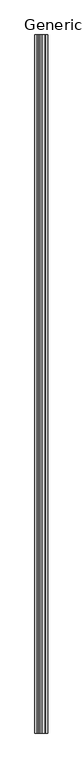
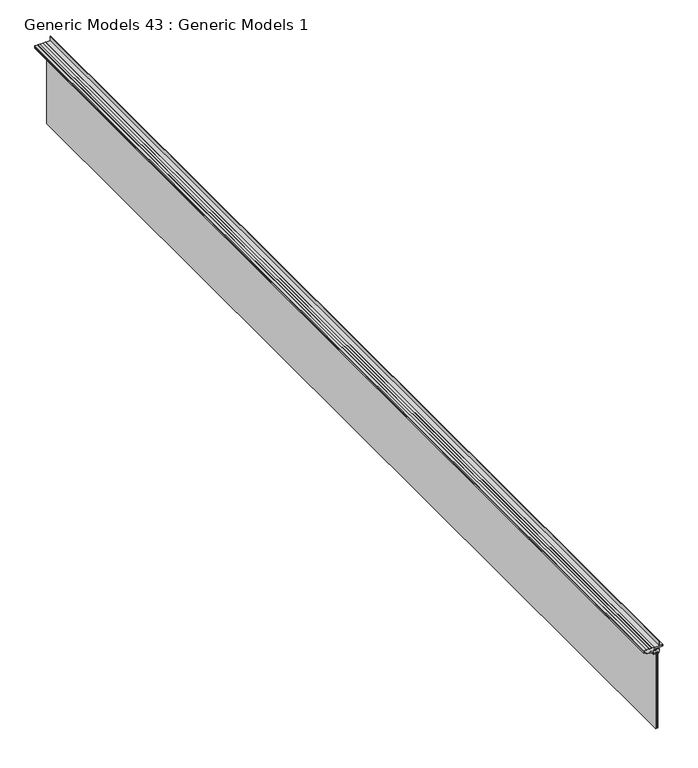
"""IFC4 building model written with IfcOpenShell, lengths in millimetres: proxy geometry, Generic Models 43 : Generic Models 1."""

from ifc_helpers import new_model, si_unit, point, frame, frame_2d, origin, place, context, project, spatial, polyline, circle_curve, trimmed, segment, composite_curve, outline, extrude, source, transform, mapped, element, save


def generic_models_43_generic_models_1_91aa61af(model_context):
    return source(origin(), model_context, "Body", "SweptSolid", [
        extrude(outline(composite_curve([segment(polyline([(126196.7118395, 4830.4400913), (126188.7616223, 4830.4400913), (126188.7616223, 4838.3902843), (126186.7804448, 4838.3902843), (126186.7804448, 4830.4400913), (126176.8490258, 4830.4400913), (126176.8490258, 4840.7524463), (126176.0362363, 4841.5398982), (126176.0362363, 4844.7148982), (126172.0738328, 4844.7148982), (126172.0738328, 4846.3150913), (126168.8988328, 4850.2520602), (126168.8988328, 4851.8522533), (126166.5112363, 4851.8522533), (126166.5112363, 4870.9022533), (126160.1794038, 4870.9022533), (126160.1794038, 4900.3154773), (126163.3544038, 4900.3154773), (126163.3544038, 4897.2675044), (126172.0412038, 4897.2675044), (126172.0412038, 4879.7415044), (126174.3272038, 4879.7415044), (126174.3272038, 4897.2675044), (126175.2670003, 4897.2675044), (126175.2670003, 4905.6748401), (126183.2171933, 4905.6748401), (126183.2171933, 4907.6561145), (126176.7982537, 4907.6561145), (126176.7982537, 4911.6692416), (126181.6750463, 4911.6692416), (126181.6750463, 4946.6196416), (126184.0974162, 4974.4834416), (126193.0288395, 4974.4834416), (126193.0288395, 4966.579876), (126195.3148395, 4966.579876), (126195.3148395, 4972.929876), (126196.7118395, 4972.929876), (126196.7118395, 4948.0420416), (126232.0789265, 4948.0420416)]), True, "CONTINUOUS"), segment(trimmed(circle_curve(frame_2d((126232.0813862, 4947.3435419)), 0.6985041), [point((126232.0789265, 4948.0420416))], [point((126232.0837271, 4946.6450416))], False, "CARTESIAN"), True, "CONTINUOUS"), segment(polyline([(126232.0837271, 4946.6450416), (126196.7118395, 4946.6450416), (126196.7118395, 4910.1758738), (126193.5368395, 4910.1758738), (126193.5368395, 4907.8898738), (126196.7118395, 4907.8898738), (126196.7118395, 4890.7904913), (126194.6290395, 4890.7904913), (126194.6290395, 4887.6154913), (126196.7118395, 4887.6154913), (126196.7118395, 4870.5883916), (126193.5368395, 4870.5883916), (126193.5368395, 4868.3023877), (126196.7118395, 4868.3023877), (126196.7118395, 4850.7946386), (126193.5368395, 4850.7946386), (126193.5368395, 4848.5086347), (126196.7118395, 4848.5086347), (126196.7118395, 4830.4400913)]), True, "CONTINUOUS")], self_intersect=False)), frame((0.0, -1504.2676118, 0.0), z_axis=(0.0, 1.0, 0.0), x_axis=(0.0, 0.0, 1.0)), (0.0, 0.0, 1.0), 7886.7),
        extrude(outline(composite_curve([segment(polyline([(126147.8549287, 4938.1431837), (126143.6194895, 4938.1431837), (126143.6194895, 4939.2790416), (126141.5931157, 4939.2790416), (126141.7826661, 4941.7220811), (126149.5884895, 4944.2574416), (126149.5884895, 4946.6450416), (126171.8896895, 4946.6450416)]), True, "CONTINUOUS"), segment(trimmed(circle_curve(frame_2d((126171.8896895, 4944.2574416)), 2.3876), [point((126171.8896895, 4946.6450416))], [point((126174.2772895, 4944.2574416))], False, "CARTESIAN"), True, "CONTINUOUS"), segment(polyline([(126174.2772895, 4944.2574416), (126174.2772895, 4941.6920416), (126172.2452895, 4941.6920416), (126172.2452895, 4940.0156416), (126168.9432895, 4940.0156416), (126168.9432895, 4938.1106416), (126176.8680895, 4938.1106416), (126176.8680895, 4932.4972416), (126171.5594895, 4932.4972416), (126171.5594895, 4920.3052416)]), True, "CONTINUOUS"), segment(trimmed(circle_curve(frame_2d((126171.5594895, 4918.3240416)), 1.9812), [point((126171.5594895, 4920.3052416))], [point((126171.5594895, 4916.3428416))], True, "CARTESIAN"), True, "CONTINUOUS"), segment(polyline([(126171.5594895, 4916.3428416), (126171.5594895, 4903.0078416)]), True, "CONTINUOUS"), segment(trimmed(circle_curve(frame_2d((126170.7466895, 4903.0078416)), 0.8128), [point((126171.5594895, 4903.0078416))], [point((126170.7466895, 4902.1950416))], False, "CARTESIAN"), True, "CONTINUOUS"), segment(polyline([(126170.7466895, 4902.1950416), (126152.4586895, 4902.1950416), (126152.4586895, 4904.0755596), (126150.8578007, 4904.0755596), (126150.8578007, 4902.4753596), (126143.3140007, 4902.4753596), (126143.3140007, 4906.2432791), (126141.1516507, 4906.2432791), (126140.1390007, 4918.0709596), (126150.0704007, 4918.0709596), (126152.4586895, 4915.6826708), (126152.4586895, 4937.1200416), (126148.8780708, 4937.1200416), (126147.8549287, 4938.1431837)]), True, "CONTINUOUS")], self_intersect=False)), frame((0.0, -1504.2676118, 0.0), z_axis=(0.0, 1.0, 0.0), x_axis=(0.0, 0.0, 1.0)), (0.0, 0.0, 1.0), 7886.7),
        extrude(outline(polyline([(4923.6272096, -1504.2676118), (4918.8647096, -1504.2676118), (4918.8647096, 6382.4323882), (4923.6272096, 6382.4323882), (4923.6272096, -1504.2676118)])), frame((0.0, 0.0, 125549.3273915), z_axis=(0.0, 0.0, 1.0), x_axis=(1.0, 0.0, 0.0)), (0.0, 0.0, 1.0), 602.3375481),
        extrude(outline(polyline([(4930.7700416, -1504.2676118), (4924.4209596, -1504.2676118), (4924.4209596, 6382.4323882), (4930.7700416, 6382.4323882), (4930.7700416, -1504.2676118)])), frame((0.0, 0.0, 126145.3149395), z_axis=(0.0, 0.0, 1.0), x_axis=(1.0, 0.0, 0.0)), (0.0, 0.0, 1.0), 6.35),
        extrude(outline(polyline([(4936.3262916, -1504.2676118), (4931.5637916, -1504.2676118), (4931.5637916, 6382.4323882), (4936.3262916, 6382.4323882), (4936.3262916, -1504.2676118)])), frame((0.0, 0.0, 125549.3273915), z_axis=(0.0, 0.0, 1.0), x_axis=(1.0, 0.0, 0.0)), (0.0, 0.0, 1.0), 602.3375481),
    ])


if __name__ == "__main__":
    model = new_model("IFC4")
    model_context = context("Model", 3, world=origin())
    ifc_project = project(units=[si_unit("LENGTHUNIT", "METRE", prefix="MILLI")], contexts=[model_context])
    site = spatial("IfcSite", under=ifc_project)
    building = spatial("IfcBuilding", under=site)
    placement = place(None, origin())
    generic_models_43_generic_models_1_shape = generic_models_43_generic_models_1_91aa61af(model_context)
    element("IfcBuildingElementProxy", 1, Name="Generic Models 43 : Generic Models 1", ObjectType="Generic Models 43 : Generic Models 1", at=placement, inside=building, context=model_context, shape_type="MappedRepresentation", body=[
        mapped(generic_models_43_generic_models_1_shape, transform((0.0, 0.0, 0.0), x_axis=(1.0, 0.0, 0.0), y_axis=(0.0, 1.0, 0.0), z_axis=(0.0, 0.0, 1.0))),
    ])
    save(model, "model.ifc")

# Revit data of these elements
# Element 1 (IfcBuildingElementProxy, "Generic Models 43 : Generic Models 1")
#   Materials on its faces: "_WINDOW PER SCHEDULE"
# Materials
#   "_WINDOW PER SCHEDULE": class "Generic", colour RGB 255 255 255, transparency 0, Cost = 0
